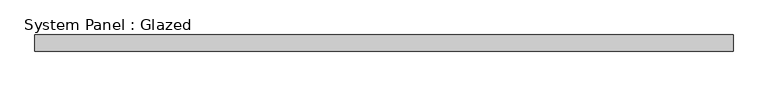
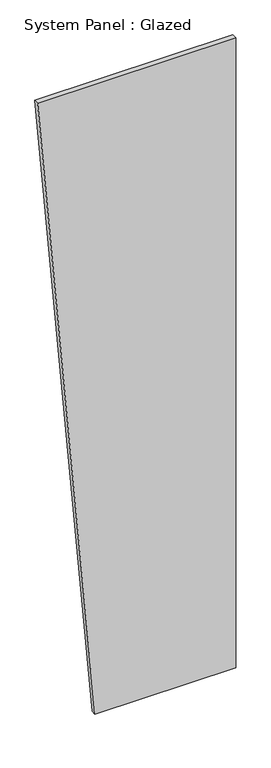
"""IFC4 building model written with IfcOpenShell, lengths in millimetres: plate geometry, System Panel : Glazed."""

from ifc_helpers import new_model, si_unit, frame, origin, place, context, project, spatial, polyline, outline, extrude, source, transform, mapped, element, save


def system_panel_glazed_d5b9b34d(model_context):
    return source(origin(), model_context, "Body", "SweptSolid", [
        extrude(outline(polyline([(0.0, -228.6), (0.0, 543.7370389), (3657.6, 543.7370389), (3657.6, -543.7370389), (0.0, -228.6)])), frame((0.0, -44.45, 0.0), z_axis=(0.0, 1.0, 0.0), x_axis=(0.0, 0.0, 1.0)), (0.0, 0.0, 1.0), 25.4),
    ])


if __name__ == "__main__":
    model = new_model("IFC4")
    model_context = context("Model", 3, world=origin())
    ifc_project = project(units=[si_unit("LENGTHUNIT", "METRE", prefix="MILLI")], contexts=[model_context])
    site = spatial("IfcSite", under=ifc_project)
    building = spatial("IfcBuilding", under=site)
    placement = place(None, origin())
    system_panel_glazed_shape = system_panel_glazed_d5b9b34d(model_context)
    element("IfcPlate", 1, ObjectType="System Panel : Glazed", at=placement, inside=building, context=model_context, shape_type="MappedRepresentation", body=[
        mapped(system_panel_glazed_shape, transform((0.0, 0.0, 0.0), x_axis=(1.0, 0.0, 0.0), y_axis=(0.0, 1.0, 0.0), z_axis=(0.0, 0.0, 1.0))),
    ])
    save(model, "model.ifc")

# Revit data of these elements
# Type "System Panel : Glazed"
#   Construction Type Id = "GSP4R"
#   Analytic Construction = "1/8 in Pilkington single glazing"
#   Visual Light Transmittance = 0.9
#   Solar Heat Gain Coefficient = 0.86
#   Heat Transfer Coefficient (U) = 1.18115 BTU/(h·ft²·°F)
#   Define Thermal Properties by = 1
# Element 1 (IfcPlate, "System Panel : Glazed")
#   Materials on its faces: "Glass"
# Materials
#   "Glass": class "Glass", colour RGB 0 128 192, transparency 0.75, Description = "Soda Lime Glass", Cost = 0
